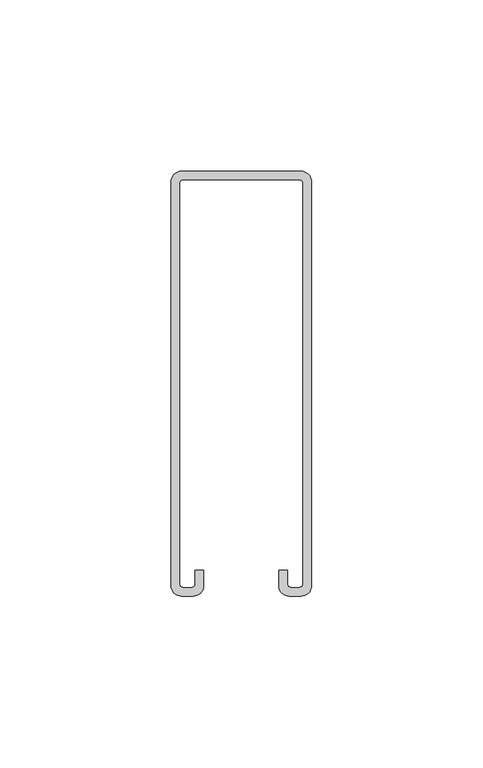
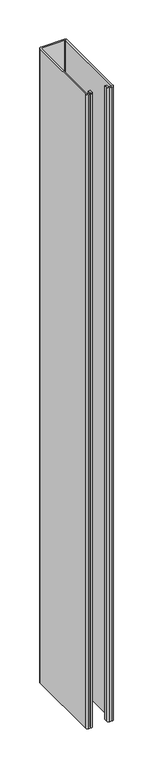
"""IFC4 building model written with IfcOpenShell, lengths in millimetres: proxy geometry, TN_Профиль монтажный : Профиль монтажный 41x124x2,5-6000."""

import ifcopenshell
import ifcopenshell.guid

model = None  # the IFC model being written
_history = None  # IfcOwnerHistory: only IFC2X3 demands one
_inside = {}  # id of a spatial element -> (the spatial element, [elements in it])
_under = {}  # id of a project, library or spatial element -> (it, [spatial elements below it])
_declared = {}  # id of a project -> (the project, [libraries it declares])
_typed = {}  # id of a type object -> (the type object, [elements of that type])
_made_of = {}  # id of a material, layer set ... -> (it, [elements and type objects made of it])


def new_model(schema):
    """Start an empty IFC model of exactly this schema.

    Asked for "IFC4X3", IfcOpenShell would pick the latest addendum, in which some entities
    have other attributes; the version numbers below select the first issue.
    IFC2X3 requires an IfcOwnerHistory on every rooted entity: one is made here for all.
    """
    global model, _history
    if schema == "IFC4X3":
        model = ifcopenshell.file(schema_version=(4, 3, 0, 0))
    else:
        model = ifcopenshell.file(schema=schema)
    _inside.clear()
    _under.clear()
    _declared.clear()
    _typed.clear()
    _made_of.clear()
    _history = None
    if model.schema == "IFC2X3":
        org = make("IfcOrganization", Name="unknown")
        user = make(
            "IfcPersonAndOrganization",
            ThePerson=make("IfcPerson", FamilyName="unknown"),
            TheOrganization=org,
        )
        app = make(
            "IfcApplication",
            ApplicationDeveloper=org,
            Version="unknown",
            ApplicationFullName="unknown",
            ApplicationIdentifier="unknown",
        )
        _history = make(
            "IfcOwnerHistory",
            OwningUser=user,
            OwningApplication=app,
            ChangeAction="ADDED",
            CreationDate=0,
        )
    return model


def make(cls, **values):
    """One entity of the class cls with the attributes given. An attribute that is None is left unset."""
    return model.create_entity(
        cls, **{name: value for name, value in values.items() if value is not None}
    )


def rooted(cls, **values):
    """An entity with a GlobalId (a new one), such as an element, a storey or a relation."""
    return make(cls, GlobalId=ifcopenshell.guid.new(), OwnerHistory=_history, **values)


def si_unit(unit_type, name, prefix=None):
    """IfcSIUnit, for example si_unit("LENGTHUNIT", "METRE", prefix="MILLI")."""
    return make("IfcSIUnit", UnitType=unit_type, Prefix=prefix, Name=name)


def assignment(units):
    """IfcUnitAssignment: the units of a project."""
    return None if units is None else make("IfcUnitAssignment", Units=units)


def point(xyz):
    """IfcCartesianPoint."""
    return None if xyz is None else make("IfcCartesianPoint", Coordinates=xyz)


def direction(xyz):
    """IfcDirection."""
    return None if xyz is None else make("IfcDirection", DirectionRatios=xyz)


def frame(location, z_axis=None, x_axis=None):
    """IfcAxis2Placement3D, a coordinate frame: its origin and axes. An axis left out is left unset."""
    return make(
        "IfcAxis2Placement3D",
        Location=point(location),
        Axis=direction(z_axis),
        RefDirection=direction(x_axis),
    )


def frame_2d(location, x_axis=None):
    """IfcAxis2Placement2D, a coordinate frame in the plane: its origin and x axis."""
    return make(
        "IfcAxis2Placement2D", Location=point(location), RefDirection=direction(x_axis)
    )


def origin():
    """The frame at (0, 0, 0) with its axes left unset."""
    return frame((0.0, 0.0, 0.0))


def origin_with_axes():
    """The frame at (0, 0, 0) with the z axis (0, 0, 1) and the x axis (1, 0, 0) written out."""
    return frame((0.0, 0.0, 0.0), z_axis=(0.0, 0.0, 1.0), x_axis=(1.0, 0.0, 0.0))


def place(relative_to, where):
    """IfcLocalPlacement: puts the frame where relative to a parent placement (None: the world)."""
    return make(
        "IfcLocalPlacement", PlacementRelTo=relative_to, RelativePlacement=where
    )


def context(
    kind, dimensions, precision=None, world=None, true_north=None, identifier=None
):
    """IfcGeometricRepresentationContext, for example the 3D "Model" context."""
    return make(
        "IfcGeometricRepresentationContext",
        ContextIdentifier=identifier,
        ContextType=kind,
        CoordinateSpaceDimension=dimensions,
        Precision=precision,
        WorldCoordinateSystem=world,
        TrueNorth=true_north,
    )


def project(units=None, contexts=None):
    """IfcProject with its units and contexts."""
    return rooted(
        "IfcProject",
        Name="project",
        RepresentationContexts=contexts,
        UnitsInContext=assignment(units),
    )


def spatial(cls, under=None, at=None, **own):
    """A site, building, storey or space (cls), placed at a placement, below another one or the project."""
    s = rooted(cls, ObjectPlacement=at, **own)
    if under is not None:
        _under.setdefault(under.id(), (under, []))[1].append(s)
    return s


def polyline(points):
    """IfcPolyline through the points."""
    return make("IfcPolyline", Points=[point(p) for p in points])


def circle_curve(where, radius):
    """IfcCircle in the frame where."""
    return make("IfcCircle", Position=where, Radius=radius)


def trimmed(basis, trim1, trim2, sense, master):
    """IfcTrimmedCurve: the piece of a basis curve between two trims."""
    return make(
        "IfcTrimmedCurve",
        BasisCurve=basis,
        Trim1=trim1,
        Trim2=trim2,
        SenseAgreement=sense,
        MasterRepresentation=master,
    )


def segment(curve, same_sense, transition):
    """IfcCompositeCurveSegment."""
    return make(
        "IfcCompositeCurveSegment",
        Transition=transition,
        SameSense=same_sense,
        ParentCurve=curve,
    )


def composite_curve(segments, self_intersect=None):
    """IfcCompositeCurve: segments joined end to end."""
    return make("IfcCompositeCurve", Segments=segments, SelfIntersect=self_intersect)


def outline(outer, holes=None, kind="AREA"):
    """IfcArbitraryClosedProfileDef: a profile drawn as a closed curve; with holes, ...WithVoids."""
    if holes is None:
        return make("IfcArbitraryClosedProfileDef", ProfileType=kind, OuterCurve=outer)
    return make(
        "IfcArbitraryProfileDefWithVoids",
        ProfileType=kind,
        OuterCurve=outer,
        InnerCurves=holes,
    )


def extrude(swept, where, along, depth):
    """IfcExtrudedAreaSolid: the profile swept, set in the frame where, extruded along a direction by depth."""
    return make(
        "IfcExtrudedAreaSolid",
        SweptArea=swept,
        Position=where,
        ExtrudedDirection=direction(along),
        Depth=depth,
    )


def shape(context_of_items, identifier, shape_type, items):
    """IfcShapeRepresentation: the items that make up one representation, for example the "Body"."""
    return make(
        "IfcShapeRepresentation",
        ContextOfItems=context_of_items,
        RepresentationIdentifier=identifier,
        RepresentationType=shape_type,
        Items=items,
    )


def source(mapping_origin, context_of_items, identifier, shape_type, items):
    """IfcRepresentationMap: a shape defined once, which mapped items show again and again."""
    return make(
        "IfcRepresentationMap",
        MappingOrigin=mapping_origin,
        MappedRepresentation=shape(context_of_items, identifier, shape_type, items),
    )


def transform(
    local_origin,
    x_axis=None,
    y_axis=None,
    z_axis=None,
    scale=None,
    scale2=None,
    scale3=None,
    uniform=True,
):
    """IfcCartesianTransformationOperator3D, or its non-uniform kind. x_axis, y_axis, z_axis: its Axis1, 2, 3."""
    if uniform:
        return make(
            "IfcCartesianTransformationOperator3D",
            Axis1=direction(x_axis),
            Axis2=direction(y_axis),
            LocalOrigin=point(local_origin),
            Scale=scale,
            Axis3=direction(z_axis),
        )
    return make(
        "IfcCartesianTransformationOperator3DnonUniform",
        Axis1=direction(x_axis),
        Axis2=direction(y_axis),
        LocalOrigin=point(local_origin),
        Scale=scale,
        Axis3=direction(z_axis),
        Scale2=scale2,
        Scale3=scale3,
    )


def mapped(mapping_source, mapping_target):
    """IfcMappedItem: shows the shape of a source again, moved by a transform."""
    return make(
        "IfcMappedItem", MappingSource=mapping_source, MappingTarget=mapping_target
    )


def made_of(thing, what):
    """Note that an element or type object is made of a material, layer set ...; save() writes the relation."""
    if what is not None:
        _made_of.setdefault(what.id(), (what, []))[1].append(thing)
    return thing


def element(
    cls,
    number,
    at=None,
    inside=None,
    cuts=None,
    type_object=None,
    material=None,
    context=None,
    identifier="Body",
    shape_type=None,
    held_by="IfcProductDefinitionShape",
    body=None,
    shapes=None,
    **own,
):
    """One element of the class cls, such as IfcWall. Its Tag is "e" and its number.

    at: its placement. inside: the storey or other place that contains it. cuts: it is an
    opening in that element (IfcRelVoidsElement). A single representation is given by context,
    identifier, shape_type and body (its items); several are given by shapes. held_by: the class
    of the entity that holds the representations. save() writes the other relations.
    """
    e = rooted(cls, Tag="e%d" % number, ObjectPlacement=at, **own)
    if body is not None:
        shapes = [shape(context, identifier, shape_type, body)]
    if shapes is not None:
        e.Representation = make(held_by, Representations=shapes)
    if inside is not None:
        _inside.setdefault(inside.id(), (inside, []))[1].append(e)
    if cuts is not None:
        rooted(
            "IfcRelVoidsElement", RelatingBuildingElement=cuts, RelatedOpeningElement=e
        )
    if type_object is not None:
        _typed.setdefault(type_object.id(), (type_object, []))[1].append(e)
    return made_of(e, material)


def aggregate(whole, parts):
    """IfcRelAggregates: a whole, such as a stair, and the parts it consists of."""
    return rooted("IfcRelAggregates", RelatingObject=whole, RelatedObjects=parts)


def save(model, path):
    """Write the relations noted so far, then the file.

    IfcRelAggregates (storeys below a building ...), IfcRelContainedInSpatialStructure (elements
    in a storey), IfcRelDefinesByType, IfcRelAssociatesMaterial and IfcRelDeclares: one each for
    every whole, place, type object, material and project.
    """
    for whole, parts in _under.values():
        aggregate(whole, parts)
    for where, things in _inside.values():
        rooted(
            "IfcRelContainedInSpatialStructure",
            RelatedElements=things,
            RelatingStructure=where,
        )
    for kind, things in _typed.values():
        rooted("IfcRelDefinesByType", RelatedObjects=things, RelatingType=kind)
    for what, things in _made_of.values():
        rooted("IfcRelAssociatesMaterial", RelatedObjects=things, RelatingMaterial=what)
    for by, libraries in _declared.values():
        rooted("IfcRelDeclares", RelatingContext=by, RelatedDefinitions=libraries)
    model.write(path)


def generic_models_741621dd(model_context):
    return source(origin(), model_context, "Body", "SweptSolid", [
        extrude(outline(composite_curve([segment(trimmed(circle_curve(frame_2d((-17.5, -3.0)), 3.0), [point((-20.5, -3.0))], [point((-17.5, 0.0))], False, "CARTESIAN"), True, "CONTINUOUS"), segment(polyline([(-17.5, 0.0), (17.5, 0.0)]), True, "CONTINUOUS"), segment(trimmed(circle_curve(frame_2d((17.5, -3.0)), 3.0), [point((17.5, 0.0))], [point((20.5, -3.0))], False, "CARTESIAN"), True, "CONTINUOUS"), segment(polyline([(20.5, -3.0), (20.5, -121.0)]), True, "CONTINUOUS"), segment(trimmed(circle_curve(frame_2d((17.5, -121.0)), 3.0), [point((20.5, -121.0))], [point((17.5, -124.0))], False, "CARTESIAN"), True, "CONTINUOUS"), segment(polyline([(17.5, -124.0), (14.0, -124.0)]), True, "CONTINUOUS"), segment(trimmed(circle_curve(frame_2d((14.0, -121.0)), 3.0), [point((14.0, -124.0))], [point((11.0, -121.0))], False, "CARTESIAN"), True, "CONTINUOUS"), segment(polyline([(11.0, -121.0), (11.0, -116.5), (13.5, -116.5), (13.5, -120.5)]), True, "CONTINUOUS"), segment(trimmed(circle_curve(frame_2d((14.5, -120.5)), 1.0), [point((13.5, -120.5))], [point((14.5, -121.5))], True, "CARTESIAN"), True, "CONTINUOUS"), segment(polyline([(14.5, -121.5), (17.0, -121.5)]), True, "CONTINUOUS"), segment(trimmed(circle_curve(frame_2d((17.0, -120.5)), 1.0), [point((17.0, -121.5))], [point((18.0, -120.5))], True, "CARTESIAN"), True, "CONTINUOUS"), segment(polyline([(18.0, -120.5), (18.0, -3.5)]), True, "CONTINUOUS"), segment(trimmed(circle_curve(frame_2d((17.0, -3.5)), 1.0), [point((18.0, -3.5))], [point((17.0, -2.5))], True, "CARTESIAN"), True, "CONTINUOUS"), segment(polyline([(17.0, -2.5), (-17.0, -2.5)]), True, "CONTINUOUS"), segment(trimmed(circle_curve(frame_2d((-17.0, -3.5)), 1.0), [point((-17.0, -2.5))], [point((-18.0, -3.5))], True, "CARTESIAN"), True, "CONTINUOUS"), segment(polyline([(-18.0, -3.5), (-18.0, -120.5)]), True, "CONTINUOUS"), segment(trimmed(circle_curve(frame_2d((-17.0, -120.5)), 1.0), [point((-18.0, -120.5))], [point((-17.0, -121.5))], True, "CARTESIAN"), True, "CONTINUOUS"), segment(polyline([(-17.0, -121.5), (-14.5, -121.5)]), True, "CONTINUOUS"), segment(trimmed(circle_curve(frame_2d((-14.5, -120.5)), 1.0), [point((-14.5, -121.5))], [point((-13.5, -120.5))], True, "CARTESIAN"), True, "CONTINUOUS"), segment(polyline([(-13.5, -120.5), (-13.5, -116.5), (-11.0, -116.5), (-11.0, -120.9588961)]), True, "CONTINUOUS"), segment(trimmed(circle_curve(frame_2d((-14.0411039, -120.9588961)), 3.0411039), [point((-11.0, -120.9588961))], [point((-14.0411039, -124.0))], False, "CARTESIAN"), True, "CONTINUOUS"), segment(polyline([(-14.0411039, -124.0), (-17.5, -124.0)]), True, "CONTINUOUS"), segment(trimmed(circle_curve(frame_2d((-17.5, -121.0)), 3.0), [point((-17.5, -124.0))], [point((-20.5, -121.0))], False, "CARTESIAN"), True, "CONTINUOUS"), segment(polyline([(-20.5, -121.0), (-20.5, -3.0)]), True, "CONTINUOUS")], self_intersect=False)), origin_with_axes(), (0.0, 0.0, 1.0), 1000.0),
    ])


if __name__ == "__main__":
    model = new_model("IFC4")
    model_context = context("Model", 3, world=origin())
    ifc_project = project(units=[si_unit("LENGTHUNIT", "METRE", prefix="MILLI")], contexts=[model_context])
    site = spatial("IfcSite", under=ifc_project)
    building = spatial("IfcBuilding", under=site)
    placement = place(None, origin())
    generic_models_shape = generic_models_741621dd(model_context)
    element("IfcBuildingElementProxy", 1, Name="TN_Профиль монтажный : Профиль монтажный 41x124x2,5-6000", ObjectType="TN_Профиль монтажный : Профиль монтажный 41x124x2,5-6000", at=placement, inside=building, context=model_context, shape_type="MappedRepresentation", body=[
        mapped(generic_models_shape, transform((0.0, 0.0, 0.0), x_axis=(1.0, 0.0, 0.0), y_axis=(0.0, 1.0, 0.0), z_axis=(0.0, 0.0, 1.0))),
    ])
    save(model, "model.ifc")

# Revit data of these elements
# Type "TN_Профиль монтажный : Профиль монтажный 41x124x2,5-6000"
#   Description = "Профиль монтажный – траверса С-образной формы предназначен для горизонтального и вертикального монтажа тяжелых инженерных систем, оборудования систем вентиляции и кондиционирования, установок электроснабжения, элементов трубопроводов, также для изготовления стенных консолей пристенного монтажа, рам оснований различного типа под оборудование. Возможно замещение на основе сконструированных модулей серийных опор ГОСТ для раскрепления технологических трубопроводов. Рекомендуется для применения в сухих, влажных помещениях и на открытом воздухе."
#   Manufacturer = "ТехноНИКОЛЬ"
#   Model = "Комплектующие к опорам"
#   URL = "https://nav.tn.ru/knowledge-base/polimernye-membrany/opory-pod-oborudovanie-na-ploskoy-krovle/?sphrase_id=266812"
#   ADSK_Обозначение = "ТехноНИКОЛЬ"
#   ADSK_Наименование краткое = "П41x124x2,5"
#   ADSK_Наименование = "Профиль монтажный 41x124x2,5-6000"
#   ADSK_Масса_Текст = ""
#   ADSK_Марка = "П41x124x2,5"
#   ADSK_Код изделия = "690881"
#   ADSK_Завод-изготовитель = "ТехноНИКОЛЬ"
#   ADSK_Единица измерения = "п.м."
#   ADSK_Группирование = "Комплектующие к опорам"
#   ADSK_URL страницы изделия = "https://nav.tn.ru/knowledge-base/polimernye-membrany/opory-pod-oborudovanie-na-ploskoy-krovle/?sphrase_id=266812"
#   ADSK_URL документации изделия = ""
#   Размер_Длина_Вводимая [instance default] = 1000 mm
#   ADSK_Размер_Длина [instance default] = 1000 mm
#   ADSK_Количество [instance default] = 1
#   Тип профиля = 2
#   Профиль монтажный 41х41x2,0 = no
#   Профиль монтажный 41x62x2,5 = no
#   Профиль монтажный 41x124x2,5 = yes
#   ADSK_Материал = TN_СтальГальванизированная_Серый
#   Default Elevation = 0
# Element 1 (IfcBuildingElementProxy, "TN_Профиль монтажный : Профиль монтажный 41x124x2,5-6000")
#   Materials on its faces: "TN_СтальГальванизированная_Серый"
# Materials
#   "TN_СтальГальванизированная_Серый": class "Типовые", colour RGB 206 210 213, transparency 0, Cost = 0
